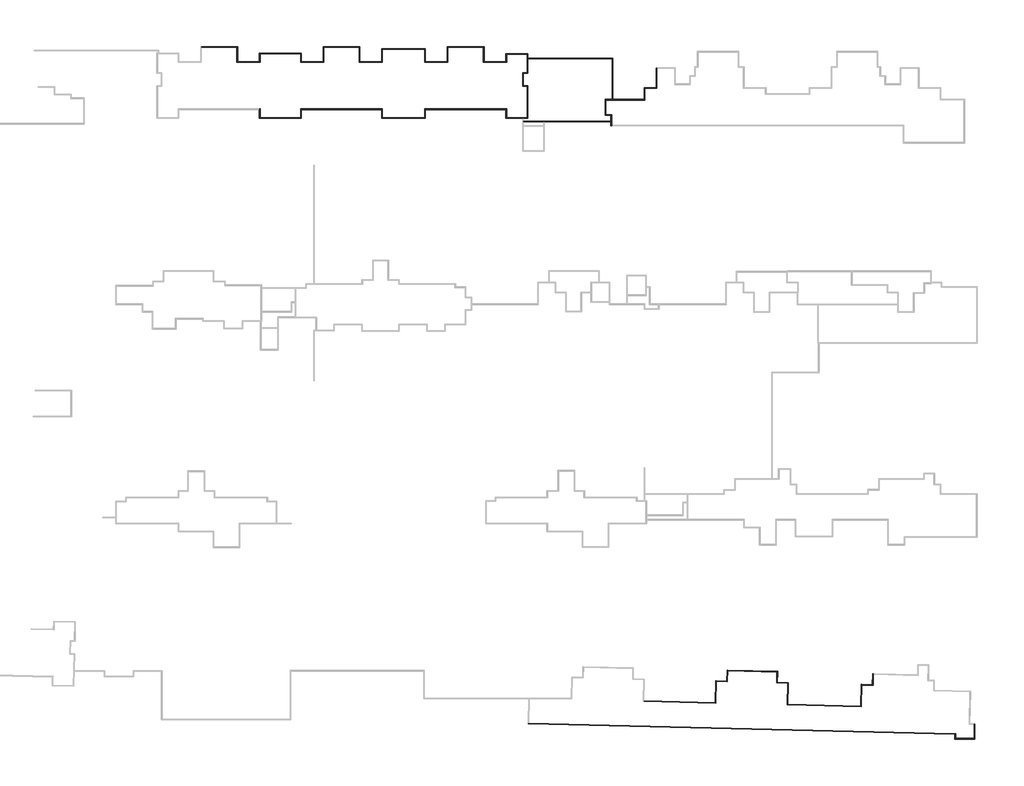
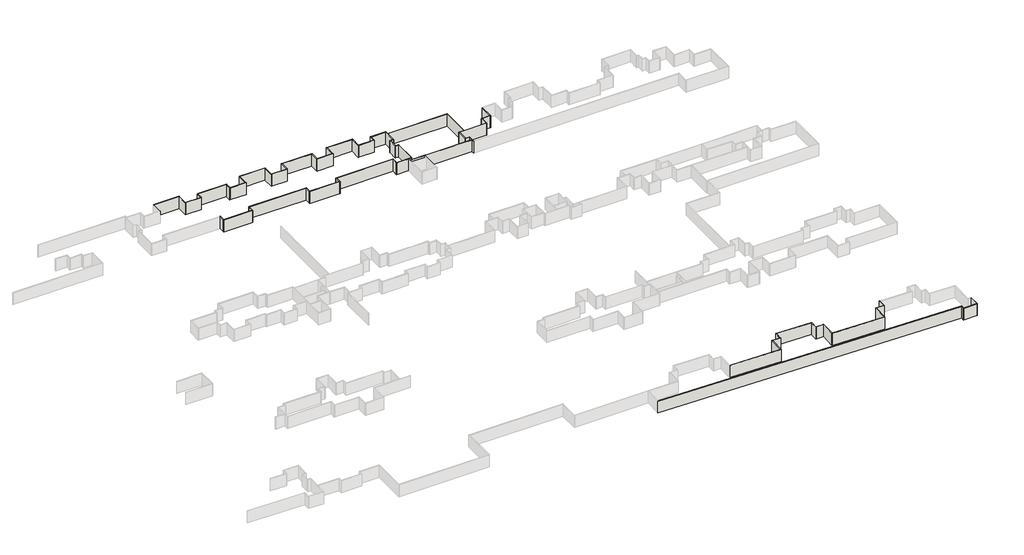
# One storey, part 6 of 8: 62 walls.
"""IFC4 building model written with IfcOpenShell, lengths in millimetres."""

import ifcopenshell
import ifcopenshell.guid

model = None  # the IFC model being written
_history = None  # IfcOwnerHistory: only IFC2X3 demands one
_inside = {}  # id of a spatial element -> (the spatial element, [elements in it])
_under = {}  # id of a project, library or spatial element -> (it, [spatial elements below it])
_declared = {}  # id of a project -> (the project, [libraries it declares])
_typed = {}  # id of a type object -> (the type object, [elements of that type])
_made_of = {}  # id of a material, layer set ... -> (it, [elements and type objects made of it])


def new_model(schema):
    """Start an empty IFC model of exactly this schema.

    Asked for "IFC4X3", IfcOpenShell would pick the latest addendum, in which some entities
    have other attributes; the version numbers below select the first issue.
    IFC2X3 requires an IfcOwnerHistory on every rooted entity: one is made here for all.
    """
    global model, _history
    if schema == "IFC4X3":
        model = ifcopenshell.file(schema_version=(4, 3, 0, 0))
    else:
        model = ifcopenshell.file(schema=schema)
    _inside.clear()
    _under.clear()
    _declared.clear()
    _typed.clear()
    _made_of.clear()
    _history = None
    if model.schema == "IFC2X3":
        org = make("IfcOrganization", Name="unknown")
        user = make(
            "IfcPersonAndOrganization",
            ThePerson=make("IfcPerson", FamilyName="unknown"),
            TheOrganization=org,
        )
        app = make(
            "IfcApplication",
            ApplicationDeveloper=org,
            Version="unknown",
            ApplicationFullName="unknown",
            ApplicationIdentifier="unknown",
        )
        _history = make(
            "IfcOwnerHistory",
            OwningUser=user,
            OwningApplication=app,
            ChangeAction="ADDED",
            CreationDate=0,
        )
    return model


def make(cls, **values):
    """One entity of the class cls with the attributes given. An attribute that is None is left unset."""
    return model.create_entity(
        cls, **{name: value for name, value in values.items() if value is not None}
    )


def rooted(cls, **values):
    """An entity with a GlobalId (a new one), such as an element, a storey or a relation."""
    return make(cls, GlobalId=ifcopenshell.guid.new(), OwnerHistory=_history, **values)


def si_unit(unit_type, name, prefix=None):
    """IfcSIUnit, for example si_unit("LENGTHUNIT", "METRE", prefix="MILLI")."""
    return make("IfcSIUnit", UnitType=unit_type, Prefix=prefix, Name=name)


def assignment(units):
    """IfcUnitAssignment: the units of a project."""
    return None if units is None else make("IfcUnitAssignment", Units=units)


def point(xyz):
    """IfcCartesianPoint."""
    return None if xyz is None else make("IfcCartesianPoint", Coordinates=xyz)


def direction(xyz):
    """IfcDirection."""
    return None if xyz is None else make("IfcDirection", DirectionRatios=xyz)


def frame(location, z_axis=None, x_axis=None):
    """IfcAxis2Placement3D, a coordinate frame: its origin and axes. An axis left out is left unset."""
    return make(
        "IfcAxis2Placement3D",
        Location=point(location),
        Axis=direction(z_axis),
        RefDirection=direction(x_axis),
    )


def origin():
    """The frame at (0, 0, 0) with its axes left unset."""
    return frame((0.0, 0.0, 0.0))


def origin_with_axes():
    """The frame at (0, 0, 0) with the z axis (0, 0, 1) and the x axis (1, 0, 0) written out."""
    return frame((0.0, 0.0, 0.0), z_axis=(0.0, 0.0, 1.0), x_axis=(1.0, 0.0, 0.0))


def place(relative_to, where):
    """IfcLocalPlacement: puts the frame where relative to a parent placement (None: the world)."""
    return make(
        "IfcLocalPlacement", PlacementRelTo=relative_to, RelativePlacement=where
    )


def context(
    kind, dimensions, precision=None, world=None, true_north=None, identifier=None
):
    """IfcGeometricRepresentationContext, for example the 3D "Model" context."""
    return make(
        "IfcGeometricRepresentationContext",
        ContextIdentifier=identifier,
        ContextType=kind,
        CoordinateSpaceDimension=dimensions,
        Precision=precision,
        WorldCoordinateSystem=world,
        TrueNorth=true_north,
    )


def project(units=None, contexts=None):
    """IfcProject with its units and contexts."""
    return rooted(
        "IfcProject",
        Name="project",
        RepresentationContexts=contexts,
        UnitsInContext=assignment(units),
    )


def spatial(cls, under=None, at=None, **own):
    """A site, building, storey or space (cls), placed at a placement, below another one or the project."""
    s = rooted(cls, ObjectPlacement=at, **own)
    if under is not None:
        _under.setdefault(under.id(), (under, []))[1].append(s)
    return s


def polyline(points):
    """IfcPolyline through the points."""
    return make("IfcPolyline", Points=[point(p) for p in points])


def outline(outer, holes=None, kind="AREA"):
    """IfcArbitraryClosedProfileDef: a profile drawn as a closed curve; with holes, ...WithVoids."""
    if holes is None:
        return make("IfcArbitraryClosedProfileDef", ProfileType=kind, OuterCurve=outer)
    return make(
        "IfcArbitraryProfileDefWithVoids",
        ProfileType=kind,
        OuterCurve=outer,
        InnerCurves=holes,
    )


def extrude(swept, where, along, depth):
    """IfcExtrudedAreaSolid: the profile swept, set in the frame where, extruded along a direction by depth."""
    return make(
        "IfcExtrudedAreaSolid",
        SweptArea=swept,
        Position=where,
        ExtrudedDirection=direction(along),
        Depth=depth,
    )


def faces_of(points, faces, orient=None, outer=None):
    """IfcFace entities. A face is a list of loops; a loop is a list of indices into points, from 0.

    orient and outer hold one flag for each loop. By default every Orientation is true, the
    first loop of a face is its IfcFaceOuterBound and the others are IfcFaceBound.
    """
    made = []
    for i, loops in enumerate(faces):
        bounds = []
        for j, loop in enumerate(loops):
            is_outer = j == 0 if outer is None else outer[i][j]
            bounds.append(
                make(
                    "IfcFaceOuterBound" if is_outer else "IfcFaceBound",
                    Bound=make("IfcPolyLoop", Polygon=[points[k] for k in loop]),
                    Orientation=True if orient is None else orient[i][j],
                )
            )
        made.append(make("IfcFace", Bounds=bounds))
    return made


def faceted_brep(points, faces, orient=None, outer=None, voids=None):
    """IfcFacetedBrep: a solid bounded by flat faces; with voids (closed shells), ...WithVoids."""
    shared = [point(p) for p in points]
    hull = make("IfcClosedShell", CfsFaces=faces_of(shared, faces, orient, outer))
    if voids is None:
        return make("IfcFacetedBrep", Outer=hull)
    return make(
        "IfcFacetedBrepWithVoids",
        Outer=hull,
        Voids=[
            make(cls, CfsFaces=faces_of(shared, fs, o, b)) for cls, fs, o, b in voids
        ],
    )


def shape(context_of_items, identifier, shape_type, items):
    """IfcShapeRepresentation: the items that make up one representation, for example the "Body"."""
    return make(
        "IfcShapeRepresentation",
        ContextOfItems=context_of_items,
        RepresentationIdentifier=identifier,
        RepresentationType=shape_type,
        Items=items,
    )


def made_of(thing, what):
    """Note that an element or type object is made of a material, layer set ...; save() writes the relation."""
    if what is not None:
        _made_of.setdefault(what.id(), (what, []))[1].append(thing)
    return thing


def element(
    cls,
    number,
    at=None,
    inside=None,
    cuts=None,
    type_object=None,
    material=None,
    context=None,
    identifier="Body",
    shape_type=None,
    held_by="IfcProductDefinitionShape",
    body=None,
    shapes=None,
    **own,
):
    """One element of the class cls, such as IfcWall. Its Tag is "e" and its number.

    at: its placement. inside: the storey or other place that contains it. cuts: it is an
    opening in that element (IfcRelVoidsElement). A single representation is given by context,
    identifier, shape_type and body (its items); several are given by shapes. held_by: the class
    of the entity that holds the representations. save() writes the other relations.
    """
    e = rooted(cls, Tag="e%d" % number, ObjectPlacement=at, **own)
    if body is not None:
        shapes = [shape(context, identifier, shape_type, body)]
    if shapes is not None:
        e.Representation = make(held_by, Representations=shapes)
    if inside is not None:
        _inside.setdefault(inside.id(), (inside, []))[1].append(e)
    if cuts is not None:
        rooted(
            "IfcRelVoidsElement", RelatingBuildingElement=cuts, RelatedOpeningElement=e
        )
    if type_object is not None:
        _typed.setdefault(type_object.id(), (type_object, []))[1].append(e)
    return made_of(e, material)


def aggregate(whole, parts):
    """IfcRelAggregates: a whole, such as a stair, and the parts it consists of."""
    return rooted("IfcRelAggregates", RelatingObject=whole, RelatedObjects=parts)


def save(model, path):
    """Write the relations noted so far, then the file.

    IfcRelAggregates (storeys below a building ...), IfcRelContainedInSpatialStructure (elements
    in a storey), IfcRelDefinesByType, IfcRelAssociatesMaterial and IfcRelDeclares: one each for
    every whole, place, type object, material and project.
    """
    for whole, parts in _under.values():
        aggregate(whole, parts)
    for where, things in _inside.values():
        rooted(
            "IfcRelContainedInSpatialStructure",
            RelatedElements=things,
            RelatingStructure=where,
        )
    for kind, things in _typed.values():
        rooted("IfcRelDefinesByType", RelatedObjects=things, RelatingType=kind)
    for what, things in _made_of.values():
        rooted("IfcRelAssociatesMaterial", RelatedObjects=things, RelatingMaterial=what)
    for by, libraries in _declared.values():
        rooted("IfcRelDeclares", RelatingContext=by, RelatedDefinitions=libraries)
    model.write(path)


model = new_model("IFC4")

# Units and contexts
model_context = context("Model", 3, world=origin())
ifc_project = project(units=[si_unit("LENGTHUNIT", "METRE", prefix="MILLI")], contexts=[model_context])

# Site, building, storey
site = spatial("IfcSite", under=ifc_project)
building = spatial("IfcBuilding", under=site)
storey = spatial("IfcBuildingStorey", under=building, Name="户型图", Elevation=0.0)

# Walls
placement = place(None, origin())
element("IfcWall", 1, ObjectType="所有墙体", at=placement, inside=storey, context=model_context, shape_type="Brep", body=[
    faceted_brep([(171910.6969649, 142127.5312689, 0.0), (178490.6969649, 142127.5312689, 0.0), (178610.6969649, 142127.5312689, 0.0), (178610.6969649, 142127.5312689, 3300.0), (178490.6969649, 142127.5312689, 3300.0), (171910.6969649, 142127.5312689, 3300.0), (171910.6969649, 142247.5312689, 0.0), (171910.6969649, 142247.5312689, 3300.0), (178610.6969649, 142247.5312689, 3300.0), (178610.6969649, 142247.5312689, 0.0)], [[[0, 1, 2, 3, 4, 5]], [[6, 7, 8, 9]], [[2, 1, 0, 6, 9]], [[5, 4, 3, 8, 7]], [[0, 5, 7, 6]], [[3, 2, 9, 8]]]),
])
element("IfcWall", 2, ObjectType="所有墙体", at=placement, inside=storey, context=model_context, shape_type="Brep", body=[
    faceted_brep([(178490.6969649, 142127.5312689, 0.0), (178490.6969649, 139327.5312675, 0.0), (178490.6969649, 139327.5312675, 3300.0), (178490.6969649, 142127.5312689, 3300.0), (178610.6969649, 142127.5312689, 0.0), (178610.6969649, 142127.5312689, 3300.0), (178610.6969649, 139447.5312675, 3300.0), (178610.6969649, 139327.5312675, 3300.0), (178610.6969649, 139327.5312675, 0.0), (178610.6969649, 139447.5312675, 0.0)], [[[0, 1, 2, 3]], [[4, 5, 6, 7, 8, 9]], [[1, 0, 4, 9, 8]], [[3, 2, 7, 6, 5]], [[0, 3, 5, 4]], [[2, 1, 8, 7]]]),
])
element("IfcWall", 3, ObjectType="所有墙体", at=placement, inside=storey, context=model_context, shape_type="Brep", body=[
    faceted_brep([(178610.6969649, 139327.5312675, 0.0), (182760.6969646, 139327.5312675, 0.0), (182760.6969646, 139327.5312675, 3300.0), (178610.6969649, 139327.5312675, 3300.0), (178610.6969649, 139447.5312675, 0.0), (178610.6969649, 139447.5312675, 3300.0), (182640.6969646, 139447.5312675, 3300.0), (182760.6969646, 139447.5312675, 3300.0), (182760.6969646, 139447.5312675, 0.0), (182640.6969646, 139447.5312675, 0.0)], [[[0, 1, 2, 3]], [[4, 5, 6, 7, 8, 9]], [[1, 0, 4, 9, 8]], [[3, 2, 7, 6, 5]], [[0, 3, 5, 4]], [[2, 1, 8, 7]]]),
])
element("IfcWall", 4, ObjectType="所有墙体", at=placement, inside=storey, context=model_context, shape_type="Brep", body=[
    faceted_brep([(182760.6969646, 139447.5312675, 0.0), (182760.6969646, 140905.0802708, 0.0), (182760.6969646, 141025.0802708, 0.0), (182760.6969646, 141025.0802708, 3300.0), (182760.6969646, 140905.0802708, 3300.0), (182760.6969646, 139447.5312675, 3300.0), (182640.6969646, 139447.5312675, 0.0), (182640.6969646, 139447.5312675, 3300.0), (182640.6969646, 141025.0802708, 3300.0), (182640.6969646, 141025.0802708, 0.0)], [[[0, 1, 2, 3, 4, 5]], [[6, 7, 8, 9]], [[2, 1, 0, 6, 9]], [[5, 4, 3, 8, 7]], [[0, 5, 7, 6]], [[3, 2, 9, 8]]]),
])
element("IfcWall", 5, ObjectType="所有墙体", at=placement, inside=storey, context=model_context, shape_type="Brep", body=[
    faceted_brep([(182760.6969646, 140905.0802708, 0.0), (190240.6969649, 140905.0802708, 0.0), (190360.6969649, 140905.0802708, 0.0), (190360.6969649, 140905.0802708, 3300.0), (190240.6969649, 140905.0802708, 3300.0), (182760.6969646, 140905.0802708, 3300.0), (182760.6969646, 141025.0802708, 0.0), (182760.6969646, 141025.0802708, 3300.0), (190360.6969649, 141025.0802708, 3300.0), (190360.6969649, 141025.0802708, 0.0)], [[[0, 1, 2, 3, 4, 5]], [[6, 7, 8, 9]], [[2, 1, 0, 6, 9]], [[5, 4, 3, 8, 7]], [[0, 5, 7, 6]], [[3, 2, 9, 8]]]),
])
element("IfcWall", 6, ObjectType="所有墙体", at=placement, inside=storey, context=model_context, shape_type="Brep", body=[
    faceted_brep([(190240.6969649, 140905.0802708, 0.0), (190240.6969649, 139327.5312675, 0.0), (190240.6969649, 139327.5312675, 3300.0), (190240.6969649, 140905.0802708, 3300.0), (190360.6969649, 140905.0802708, 0.0), (190360.6969649, 140905.0802708, 3300.0), (190360.6969649, 139447.5312675, 3300.0), (190360.6969649, 139327.5312675, 3300.0), (190360.6969649, 139327.5312675, 0.0), (190360.6969649, 139447.5312675, 0.0)], [[[0, 1, 2, 3]], [[4, 5, 6, 7, 8, 9]], [[1, 0, 4, 9, 8]], [[3, 2, 7, 6, 5]], [[0, 3, 5, 4]], [[2, 1, 8, 7]]]),
])
element("IfcWall", 7, ObjectType="所有墙体", at=placement, inside=storey, context=model_context, shape_type="Brep", body=[
    faceted_brep([(190360.6969649, 139327.5312675, 0.0), (194510.6969649, 139327.5312675, 0.0), (194510.6969649, 139327.5312675, 3300.0), (190360.6969649, 139327.5312675, 3300.0), (190360.6969649, 139447.5312675, 0.0), (190360.6969649, 139447.5312675, 3300.0), (194390.6969649, 139447.5312675, 3300.0), (194510.6969649, 139447.5312675, 3300.0), (194510.6969649, 139447.5312675, 0.0), (194390.6969649, 139447.5312675, 0.0)], [[[0, 1, 2, 3]], [[4, 5, 6, 7, 8, 9]], [[1, 0, 4, 9, 8]], [[3, 2, 7, 6, 5]], [[0, 3, 5, 4]], [[2, 1, 8, 7]]]),
])
element("IfcWall", 8, ObjectType="所有墙体", at=placement, inside=storey, context=model_context, shape_type="Brep", body=[
    faceted_brep([(194510.6969649, 139447.5312675, 0.0), (194510.6969649, 142127.5312689, 0.0), (194510.6969649, 142247.5312689, 0.0), (194510.6969649, 142247.5312689, 3300.0), (194510.6969649, 142127.5312689, 3300.0), (194510.6969649, 139447.5312675, 3300.0), (194390.6969649, 139447.5312675, 0.0), (194390.6969649, 139447.5312675, 3300.0), (194390.6969649, 142247.5312689, 3300.0), (194390.6969649, 142247.5312689, 0.0)], [[[0, 1, 2, 3, 4, 5]], [[6, 7, 8, 9]], [[2, 1, 0, 6, 9]], [[5, 4, 3, 8, 7]], [[0, 5, 7, 6]], [[3, 2, 9, 8]]]),
])
element("IfcWall", 9, ObjectType="所有墙体", at=placement, inside=storey, context=model_context, shape_type="Brep", body=[
    faceted_brep([(194510.6969649, 142127.5312689, 0.0), (201090.6969649, 142127.5312689, 0.0), (201210.6969649, 142127.5312689, 0.0), (201210.6969649, 142127.5312689, 3300.0), (201090.6969649, 142127.5312689, 3300.0), (194510.6969649, 142127.5312689, 3300.0), (194510.6969649, 142247.5312689, 0.0), (194510.6969649, 142247.5312689, 3300.0), (201210.6969649, 142247.5312689, 3300.0), (201210.6969649, 142247.5312689, 0.0)], [[[0, 1, 2, 3, 4, 5]], [[6, 7, 8, 9]], [[2, 1, 0, 6, 9]], [[5, 4, 3, 8, 7]], [[0, 5, 7, 6]], [[3, 2, 9, 8]]]),
])
element("IfcWall", 10, ObjectType="所有墙体", at=placement, inside=storey, context=model_context, shape_type="Brep", body=[
    faceted_brep([(201090.6969649, 142127.5312689, 0.0), (201090.6969649, 139327.5312675, 0.0), (201090.6969649, 139327.5312675, 3300.0), (201090.6969649, 142127.5312689, 3300.0), (201210.6969649, 142127.5312689, 0.0), (201210.6969649, 142127.5312689, 3300.0), (201210.6969649, 139447.5312675, 3300.0), (201210.6969649, 139327.5312675, 3300.0), (201210.6969649, 139327.5312675, 0.0), (201210.6969649, 139447.5312675, 0.0)], [[[0, 1, 2, 3]], [[4, 5, 6, 7, 8, 9]], [[1, 0, 4, 9, 8]], [[3, 2, 7, 6, 5]], [[0, 3, 5, 4]], [[2, 1, 8, 7]]]),
])
element("IfcWall", 11, ObjectType="所有墙体", at=placement, inside=storey, context=model_context, shape_type="Brep", body=[
    faceted_brep([(201210.6969649, 139327.5312675, 0.0), (205360.6969646, 139327.5312675, 0.0), (205360.6969646, 139327.5312675, 3300.0), (201210.6969649, 139327.5312675, 3300.0), (201210.6969649, 139447.5312675, 0.0), (201210.6969649, 139447.5312675, 3300.0), (205240.6969646, 139447.5312675, 3300.0), (205360.6969646, 139447.5312675, 3300.0), (205360.6969646, 139447.5312675, 0.0), (205240.6969646, 139447.5312675, 0.0)], [[[0, 1, 2, 3]], [[4, 5, 6, 7, 8, 9]], [[1, 0, 4, 9, 8]], [[3, 2, 7, 6, 5]], [[0, 3, 5, 4]], [[2, 1, 8, 7]]]),
])
element("IfcWall", 12, ObjectType="所有墙体", at=placement, inside=storey, context=model_context, shape_type="Brep", body=[
    faceted_brep([(205360.6969646, 139447.5312675, 0.0), (205360.6969646, 141727.5312675, 0.0), (205360.6969646, 141847.5312675, 0.0), (205360.6969646, 141847.5312675, 3300.0), (205360.6969646, 141727.5312675, 3300.0), (205360.6969646, 139447.5312675, 3300.0), (205240.6969646, 139447.5312675, 0.0), (205240.6969646, 139447.5312675, 3300.0), (205240.6969646, 141847.5312675, 3300.0), (205240.6969646, 141847.5312675, 0.0)], [[[0, 1, 2, 3, 4, 5]], [[6, 7, 8, 9]], [[2, 1, 0, 6, 9]], [[5, 4, 3, 8, 7]], [[0, 5, 7, 6]], [[3, 2, 9, 8]]]),
])
element("IfcWall", 13, ObjectType="所有墙体", at=placement, inside=storey, context=model_context, shape_type="Brep", body=[
    faceted_brep([(205360.6969646, 141727.5312675, 0.0), (213140.6969649, 141727.5312675, 0.0), (213260.6969649, 141727.5312675, 0.0), (213260.6969649, 141727.5312675, 3300.0), (213140.6969649, 141727.5312675, 3300.0), (205360.6969646, 141727.5312675, 3300.0), (205360.6969646, 141847.5312675, 0.0), (205360.6969646, 141847.5312675, 3300.0), (213260.6969649, 141847.5312675, 3300.0), (213260.6969649, 141847.5312675, 0.0)], [[[0, 1, 2, 3, 4, 5]], [[6, 7, 8, 9]], [[2, 1, 0, 6, 9]], [[5, 4, 3, 8, 7]], [[0, 5, 7, 6]], [[3, 2, 9, 8]]]),
])
element("IfcWall", 14, ObjectType="所有墙体", at=placement, inside=storey, context=model_context, shape_type="Brep", body=[
    faceted_brep([(213140.6969649, 141727.5312675, 0.0), (213140.6969649, 139327.5312675, 0.0), (213140.6969649, 139327.5312675, 3300.0), (213140.6969649, 141727.5312675, 3300.0), (213260.6969649, 141727.5312675, 0.0), (213260.6969649, 141727.5312675, 3300.0), (213260.6969649, 139447.5312675, 3300.0), (213260.6969649, 139327.5312675, 3300.0), (213260.6969649, 139327.5312675, 0.0), (213260.6969649, 139447.5312675, 0.0)], [[[0, 1, 2, 3]], [[4, 5, 6, 7, 8, 9]], [[1, 0, 4, 9, 8]], [[3, 2, 7, 6, 5]], [[0, 3, 5, 4]], [[2, 1, 8, 7]]]),
])
element("IfcWall", 15, ObjectType="所有墙体", at=placement, inside=storey, context=model_context, shape_type="Brep", body=[
    faceted_brep([(213260.6969649, 139327.5312675, 0.0), (217410.6969649, 139327.5312675, 0.0), (217410.6969649, 139327.5312675, 3300.0), (213260.6969649, 139327.5312675, 3300.0), (213260.6969649, 139447.5312675, 0.0), (213260.6969649, 139447.5312675, 3300.0), (217290.6969649, 139447.5312675, 3300.0), (217410.6969649, 139447.5312675, 3300.0), (217410.6969649, 139447.5312675, 0.0), (217290.6969649, 139447.5312675, 0.0)], [[[0, 1, 2, 3]], [[4, 5, 6, 7, 8, 9]], [[1, 0, 4, 9, 8]], [[3, 2, 7, 6, 5]], [[0, 3, 5, 4]], [[2, 1, 8, 7]]]),
])
element("IfcWall", 16, ObjectType="所有墙体", at=placement, inside=storey, context=model_context, shape_type="Brep", body=[
    faceted_brep([(217410.6969649, 139447.5312675, 0.0), (217410.6969649, 142127.5312689, 0.0), (217410.6969649, 142247.5312689, 0.0), (217410.6969649, 142247.5312689, 3300.0), (217410.6969649, 142127.5312689, 3300.0), (217410.6969649, 139447.5312675, 3300.0), (217290.6969649, 139447.5312675, 0.0), (217290.6969649, 139447.5312675, 3300.0), (217290.6969649, 142247.5312689, 3300.0), (217290.6969649, 142247.5312689, 0.0)], [[[0, 1, 2, 3, 4, 5]], [[6, 7, 8, 9]], [[2, 1, 0, 6, 9]], [[5, 4, 3, 8, 7]], [[0, 5, 7, 6]], [[3, 2, 9, 8]]]),
])
element("IfcWall", 17, ObjectType="所有墙体", at=placement, inside=storey, context=model_context, shape_type="Brep", body=[
    faceted_brep([(217410.6969649, 142127.5312689, 0.0), (223990.6969649, 142127.5312689, 0.0), (224110.6969649, 142127.5312689, 0.0), (224110.6969649, 142127.5312689, 3300.0), (223990.6969649, 142127.5312689, 3300.0), (217410.6969649, 142127.5312689, 3300.0), (217410.6969649, 142247.5312689, 0.0), (217410.6969649, 142247.5312689, 3300.0), (224110.6969649, 142247.5312689, 3300.0), (224110.6969649, 142247.5312689, 0.0)], [[[0, 1, 2, 3, 4, 5]], [[6, 7, 8, 9]], [[2, 1, 0, 6, 9]], [[5, 4, 3, 8, 7]], [[0, 5, 7, 6]], [[3, 2, 9, 8]]]),
])
element("IfcWall", 18, ObjectType="所有墙体", at=placement, inside=storey, context=model_context, shape_type="Brep", body=[
    faceted_brep([(223990.6969649, 142127.5312689, 0.0), (223990.6969649, 139327.5312675, 0.0), (223990.6969649, 139327.5312675, 3300.0), (223990.6969649, 142127.5312689, 3300.0), (224110.6969649, 142127.5312689, 0.0), (224110.6969649, 142127.5312689, 3300.0), (224110.6969649, 139447.5312675, 3300.0), (224110.6969649, 139327.5312675, 3300.0), (224110.6969649, 139327.5312675, 0.0), (224110.6969649, 139447.5312675, 0.0)], [[[0, 1, 2, 3]], [[4, 5, 6, 7, 8, 9]], [[1, 0, 4, 9, 8]], [[3, 2, 7, 6, 5]], [[0, 3, 5, 4]], [[2, 1, 8, 7]]]),
])
element("IfcWall", 19, ObjectType="所有墙体", at=placement, inside=storey, context=model_context, shape_type="Brep", body=[
    faceted_brep([(224110.6969649, 139327.5312675, 0.0), (228260.6969646, 139327.5312675, 0.0), (228260.6969646, 139327.5312675, 3300.0), (224110.6969649, 139327.5312675, 3300.0), (224110.6969649, 139447.5312675, 0.0), (224110.6969649, 139447.5312675, 3300.0), (228140.6969646, 139447.5312675, 3300.0), (228260.6969646, 139447.5312675, 3300.0), (228260.6969646, 139447.5312675, 0.0), (228140.6969646, 139447.5312675, 0.0)], [[[0, 1, 2, 3]], [[4, 5, 6, 7, 8, 9]], [[1, 0, 4, 9, 8]], [[3, 2, 7, 6, 5]], [[0, 3, 5, 4]], [[2, 1, 8, 7]]]),
])
element("IfcWall", 20, ObjectType="所有墙体", at=placement, inside=storey, context=model_context, shape_type="Brep", body=[
    faceted_brep([(228260.6969646, 139447.5312675, 0.0), (228260.6969646, 140827.5312675, 0.0), (228260.6969646, 140947.5312675, 0.0), (228260.6969646, 140947.5312675, 3300.0), (228260.6969646, 140827.5312675, 3300.0), (228260.6969646, 139447.5312675, 3300.0), (228140.6969646, 139447.5312675, 0.0), (228140.6969646, 139447.5312675, 3300.0), (228140.6969646, 140947.5312675, 3300.0), (228140.6969646, 140947.5312675, 0.0)], [[[0, 1, 2, 3, 4, 5]], [[6, 7, 8, 9]], [[2, 1, 0, 6, 9]], [[5, 4, 3, 8, 7]], [[0, 5, 7, 6]], [[3, 2, 9, 8]]]),
])
element("IfcWall", 21, ObjectType="所有墙体", at=placement, inside=storey, context=model_context, shape_type="Brep", body=[
    faceted_brep([(228260.6969646, 140827.5312675, 0.0), (232040.6969642, 140827.5312675, 0.0), (232160.6969642, 140827.5312675, 0.0), (232160.6969642, 140827.5312675, 3300.0), (232040.6969642, 140827.5312675, 3300.0), (228260.6969646, 140827.5312675, 3300.0), (228260.6969646, 140947.5312675, 0.0), (228260.6969646, 140947.5312675, 3300.0), (232160.6969642, 140947.5312675, 3300.0), (232160.6969642, 140947.5312675, 0.0)], [[[0, 1, 2, 3, 4, 5]], [[6, 7, 8, 9]], [[2, 1, 0, 6, 9]], [[5, 4, 3, 8, 7]], [[0, 5, 7, 6]], [[3, 2, 9, 8]]]),
])
element("IfcWall", 22, ObjectType="所有墙体", at=placement, inside=storey, context=model_context, shape_type="Brep", body=[
    faceted_brep([(232040.6969642, 140827.5312675, 0.0), (232040.6969642, 137447.5312675, 0.0), (232040.6969642, 137327.5312675, 0.0), (232040.6969642, 137327.5312675, 3300.0), (232040.6969642, 137447.5312675, 3300.0), (232040.6969642, 140827.5312675, 3300.0), (232160.6969642, 140827.5312675, 0.0), (232160.6969642, 140827.5312675, 3300.0), (232160.6969642, 140107.5312675, 3300.0), (232160.6969642, 139987.5312675, 3300.0), (232160.6969642, 137327.5312675, 3300.0), (232160.6969642, 137327.5312675, 0.0), (232160.6969642, 139987.5312675, 0.0), (232160.6969642, 140107.5312675, 0.0)], [[[0, 1, 2, 3, 4, 5]], [[6, 7, 8, 9, 10, 11, 12, 13]], [[2, 1, 0, 6, 13, 12, 11]], [[5, 4, 3, 10, 9, 8, 7]], [[0, 5, 7, 6]], [[3, 2, 11, 10]]]),
])
element("IfcWall", 23, ObjectType="所有墙体", at=placement, inside=storey, context=model_context, shape_type="Brep", body=[
    faceted_brep([(232040.6969642, 137447.5312675, 0.0), (231240.6969648, 137447.5312675, 0.0), (231240.6969648, 137447.5312675, 3300.0), (232040.6969642, 137447.5312675, 3300.0), (232040.6969642, 137327.5312675, 0.0), (232040.6969642, 137327.5312675, 3300.0), (231360.6969648, 137327.5312675, 3300.0), (231240.6969648, 137327.5312675, 3300.0), (231240.6969648, 137327.5312675, 0.0), (231360.6969648, 137327.5312675, 0.0)], [[[0, 1, 2, 3]], [[4, 5, 6, 7, 8, 9]], [[1, 0, 4, 9, 8]], [[3, 2, 7, 6, 5]], [[0, 3, 5, 4]], [[2, 1, 8, 7]]]),
])
element("IfcWall", 24, ObjectType="所有墙体", at=placement, inside=storey, context=model_context, shape_type="Brep", body=[
    faceted_brep([(231240.6969648, 137327.5312675, 0.0), (231240.6969648, 134927.5312611, 0.0), (231240.6969648, 134927.5312611, 3300.0), (231240.6969648, 137327.5312675, 3300.0), (231360.6969648, 137327.5312675, 0.0), (231360.6969648, 137327.5312675, 3300.0), (231360.6969648, 135047.5312611, 3300.0), (231360.6969648, 134927.5312611, 3300.0), (231360.6969648, 134927.5312611, 0.0), (231360.6969648, 135047.5312611, 0.0)], [[[0, 1, 2, 3]], [[4, 5, 6, 7, 8, 9]], [[1, 0, 4, 9, 8]], [[3, 2, 7, 6, 5]], [[0, 3, 5, 4]], [[2, 1, 8, 7]]]),
])
element("IfcWall", 25, ObjectType="所有墙体", at=placement, inside=storey, context=model_context, shape_type="Brep", body=[
    faceted_brep([(231360.6969648, 134927.5312611, 0.0), (232040.6969642, 134927.5312611, 0.0), (232160.6969642, 134927.5312611, 0.0), (232160.6969642, 134927.5312611, 3300.0), (232040.6969642, 134927.5312611, 3300.0), (231360.6969648, 134927.5312611, 3300.0), (231360.6969648, 135047.5312611, 0.0), (231360.6969648, 135047.5312611, 3300.0), (232160.6969642, 135047.5312611, 3300.0), (232160.6969642, 135047.5312611, 0.0)], [[[0, 1, 2, 3, 4, 5]], [[6, 7, 8, 9]], [[2, 1, 0, 6, 9]], [[5, 4, 3, 8, 7]], [[0, 5, 7, 6]], [[3, 2, 9, 8]]]),
])
element("IfcWall", 26, ObjectType="所有墙体", at=placement, inside=storey, context=model_context, shape_type="Brep", body=[
    faceted_brep([(232040.6969642, 134927.5312611, 0.0), (232040.6969642, 129147.5312684, 0.0), (232040.6969642, 129027.5312684, 0.0), (232040.6969642, 129027.5312684, 3300.0), (232040.6969642, 129147.5312684, 3300.0), (232040.6969642, 134927.5312611, 3300.0), (232160.6969642, 134927.5312611, 0.0), (232160.6969642, 134927.5312611, 3300.0), (232160.6969642, 129027.5312684, 3300.0), (232160.6969642, 129027.5312684, 0.0)], [[[0, 1, 2, 3, 4, 5]], [[6, 7, 8, 9]], [[2, 1, 0, 6, 9]], [[5, 4, 3, 8, 7]], [[0, 5, 7, 6]], [[3, 2, 9, 8]]]),
])
element("IfcWall", 27, ObjectType="所有墙体", at=placement, inside=storey, context=model_context, shape_type="Brep", body=[
    faceted_brep([(232040.6969642, 129147.5312684, 0.0), (228260.6969646, 129147.5312684, 0.0), (228140.6969646, 129147.5312684, 0.0), (228140.6969646, 129147.5312684, 3300.0), (228260.6969646, 129147.5312684, 3300.0), (232040.6969642, 129147.5312684, 3300.0), (232040.6969642, 129027.5312684, 0.0), (232040.6969642, 129027.5312684, 3300.0), (231369.8041277, 129027.5312684, 3300.0), (231249.8041277, 129027.5312684, 3300.0), (228140.6969646, 129027.5312684, 3300.0), (228140.6969646, 129027.5312684, 0.0), (231249.8041277, 129027.5312684, 0.0), (231369.8041277, 129027.5312684, 0.0)], [[[0, 1, 2, 3, 4, 5]], [[6, 7, 8, 9, 10, 11, 12, 13]], [[2, 1, 0, 6, 13, 12, 11]], [[5, 4, 3, 10, 9, 8, 7]], [[0, 5, 7, 6]], [[3, 2, 11, 10]]]),
])
element("IfcWall", 28, ObjectType="所有墙体", at=placement, inside=storey, context=model_context, shape_type="Brep", body=[
    faceted_brep([(228260.6969646, 129147.5312684, 0.0), (228260.6969646, 130747.5312684, 0.0), (228260.6969646, 130747.5312684, 3300.0), (228260.6969646, 129147.5312684, 3300.0), (228140.6969646, 129147.5312684, 0.0), (228140.6969646, 129147.5312684, 3300.0), (228140.6969646, 130627.5312684, 3300.0), (228140.6969646, 130747.5312684, 3300.0), (228140.6969646, 130747.5312684, 0.0), (228140.6969646, 130627.5312684, 0.0)], [[[0, 1, 2, 3]], [[4, 5, 6, 7, 8, 9]], [[1, 0, 4, 9, 8]], [[3, 2, 7, 6, 5]], [[0, 3, 5, 4]], [[2, 1, 8, 7]]]),
])
element("IfcWall", 29, ObjectType="所有墙体", at=placement, inside=storey, context=model_context, shape_type="Brep", body=[
    faceted_brep([(228140.6969646, 130747.5312684, 0.0), (213140.6969649, 130747.5312684, 0.0), (213140.6969649, 130747.5312684, 3300.0), (228140.6969646, 130747.5312684, 3300.0), (228140.6969646, 130627.5312684, 0.0), (228140.6969646, 130627.5312684, 3300.0), (213260.6969649, 130627.5312684, 3300.0), (213140.6969649, 130627.5312684, 3300.0), (213140.6969649, 130627.5312684, 0.0), (213260.6969649, 130627.5312684, 0.0)], [[[0, 1, 2, 3]], [[4, 5, 6, 7, 8, 9]], [[1, 0, 4, 9, 8]], [[3, 2, 7, 6, 5]], [[0, 3, 5, 4]], [[2, 1, 8, 7]]]),
])
element("IfcWall", 30, ObjectType="所有墙体", at=placement, inside=storey, context=model_context, shape_type="Brep", body=[
    faceted_brep([(213140.6969649, 130627.5312684, 0.0), (213140.6969649, 129147.5312684, 0.0), (213140.6969649, 129027.5312684, 0.0), (213140.6969649, 129027.5312684, 3300.0), (213140.6969649, 129147.5312684, 3300.0), (213140.6969649, 130627.5312684, 3300.0), (213260.6969649, 130627.5312684, 0.0), (213260.6969649, 130627.5312684, 3300.0), (213260.6969649, 129027.5312684, 3300.0), (213260.6969649, 129027.5312684, 0.0)], [[[0, 1, 2, 3, 4, 5]], [[6, 7, 8, 9]], [[2, 1, 0, 6, 9]], [[5, 4, 3, 8, 7]], [[0, 5, 7, 6]], [[3, 2, 9, 8]]]),
])
element("IfcWall", 31, ObjectType="所有墙体", at=placement, inside=storey, context=model_context, shape_type="Brep", body=[
    faceted_brep([(213140.6969649, 129147.5312684, 0.0), (205360.6969646, 129147.5312684, 0.0), (205240.6969646, 129147.5312684, 0.0), (205240.6969646, 129147.5312684, 3300.0), (205360.6969646, 129147.5312684, 3300.0), (213140.6969649, 129147.5312684, 3300.0), (213140.6969649, 129027.5312684, 0.0), (213140.6969649, 129027.5312684, 3300.0), (205240.6969646, 129027.5312684, 3300.0), (205240.6969646, 129027.5312684, 0.0)], [[[0, 1, 2, 3, 4, 5]], [[6, 7, 8, 9]], [[2, 1, 0, 6, 9]], [[5, 4, 3, 8, 7]], [[0, 5, 7, 6]], [[3, 2, 9, 8]]]),
])
element("IfcWall", 32, ObjectType="所有墙体", at=placement, inside=storey, context=model_context, shape_type="Brep", body=[
    faceted_brep([(205360.6969646, 129147.5312684, 0.0), (205360.6969646, 130747.5312684, 0.0), (205360.6969646, 130747.5312684, 3300.0), (205360.6969646, 129147.5312684, 3300.0), (205240.6969646, 129147.5312684, 0.0), (205240.6969646, 129147.5312684, 3300.0), (205240.6969646, 130627.5312684, 3300.0), (205240.6969646, 130747.5312684, 3300.0), (205240.6969646, 130747.5312684, 0.0), (205240.6969646, 130627.5312684, 0.0)], [[[0, 1, 2, 3]], [[4, 5, 6, 7, 8, 9]], [[1, 0, 4, 9, 8]], [[3, 2, 7, 6, 5]], [[0, 3, 5, 4]], [[2, 1, 8, 7]]]),
])
element("IfcWall", 33, ObjectType="所有墙体", at=placement, inside=storey, context=model_context, shape_type="Brep", body=[
    faceted_brep([(205240.6969646, 130747.5312684, 0.0), (190240.6969649, 130747.5312684, 0.0), (190240.6969649, 130747.5312684, 3300.0), (205240.6969646, 130747.5312684, 3300.0), (205240.6969646, 130627.5312684, 0.0), (205240.6969646, 130627.5312684, 3300.0), (190360.6969649, 130627.5312684, 3300.0), (190240.6969649, 130627.5312684, 3300.0), (190240.6969649, 130627.5312684, 0.0), (190360.6969649, 130627.5312684, 0.0)], [[[0, 1, 2, 3]], [[4, 5, 6, 7, 8, 9]], [[1, 0, 4, 9, 8]], [[3, 2, 7, 6, 5]], [[0, 3, 5, 4]], [[2, 1, 8, 7]]]),
])
element("IfcWall", 34, ObjectType="所有墙体", at=placement, inside=storey, context=model_context, shape_type="Brep", body=[
    faceted_brep([(190240.6969649, 130627.5312684, 0.0), (190240.6969649, 129147.5312684, 0.0), (190240.6969649, 129027.5312684, 0.0), (190240.6969649, 129027.5312684, 3300.0), (190240.6969649, 129147.5312684, 3300.0), (190240.6969649, 130627.5312684, 3300.0), (190360.6969649, 130627.5312684, 0.0), (190360.6969649, 130627.5312684, 3300.0), (190360.6969649, 129027.5312684, 3300.0), (190360.6969649, 129027.5312684, 0.0)], [[[0, 1, 2, 3, 4, 5]], [[6, 7, 8, 9]], [[2, 1, 0, 6, 9]], [[5, 4, 3, 8, 7]], [[0, 5, 7, 6]], [[3, 2, 9, 8]]]),
])
element("IfcWall", 35, ObjectType="所有墙体", at=placement, inside=storey, context=model_context, shape_type="Brep", body=[
    faceted_brep([(190240.6969649, 129147.5312684, 0.0), (182760.6969646, 129147.5312684, 0.0), (182640.6969646, 129147.5312684, 0.0), (182640.6969646, 129147.5312684, 3300.0), (182760.6969646, 129147.5312684, 3300.0), (190240.6969649, 129147.5312684, 3300.0), (190240.6969649, 129027.5312684, 0.0), (190240.6969649, 129027.5312684, 3300.0), (182640.6969646, 129027.5312684, 3300.0), (182640.6969646, 129027.5312684, 0.0)], [[[0, 1, 2, 3, 4, 5]], [[6, 7, 8, 9]], [[2, 1, 0, 6, 9]], [[5, 4, 3, 8, 7]], [[0, 5, 7, 6]], [[3, 2, 9, 8]]]),
])
element("IfcWall", 36, ObjectType="所有墙体", at=placement, inside=storey, context=model_context, shape_type="Brep", body=[
    faceted_brep([(182760.6969646, 129147.5312684, 0.0), (182760.6969646, 130747.5312684, 0.0), (182760.6969646, 130747.5312684, 3300.0), (182760.6969646, 129147.5312684, 3300.0), (182640.6969646, 129147.5312684, 0.0), (182640.6969646, 129147.5312684, 3300.0), (182640.6969646, 130627.5312684, 3300.0), (182640.6969646, 130747.5312684, 3300.0), (182640.6969646, 130747.5312684, 0.0), (182640.6969646, 130627.5312684, 0.0)], [[[0, 1, 2, 3]], [[4, 5, 6, 7, 8, 9]], [[1, 0, 4, 9, 8]], [[3, 2, 7, 6, 5]], [[0, 3, 5, 4]], [[2, 1, 8, 7]]]),
])
element("IfcWall", 37, ObjectType="所有墙体", at=placement, inside=storey, context=model_context, shape_type="Brep", body=[
    faceted_brep([(253581.2528793, 21363.7654177, 0.0), (266877.2414257, 21037.1332476, 0.0), (266877.2414257, 21037.1332476, 3300.0), (253581.2528793, 21363.7654177, 3300.0), (253584.1999365, 21483.7292241, 0.0), (253584.1999365, 21483.7292241, 3300.0), (266760.2246764, 21160.0441112, 3300.0), (266880.1884829, 21157.097054, 3300.0), (266880.1884829, 21157.097054, 0.0), (266760.2246764, 21160.0441112, 0.0)], [[[0, 1, 2, 3]], [[4, 5, 6, 7, 8, 9]], [[1, 0, 4, 9, 8]], [[3, 2, 7, 6, 5]], [[0, 3, 5, 4]], [[2, 1, 8, 7]]]),
])
element("IfcWall", 38, ObjectType="所有墙体", at=placement, inside=storey, context=model_context, shape_type="Brep", body=[
    faceted_brep([(266880.1884829, 21157.097054, 0.0), (266975.9558887, 25055.4342273, 0.0), (266978.9029458, 25175.3980337, 0.0), (266978.9029458, 25175.3980337, 3300.0), (266975.9558887, 25055.4342273, 3300.0), (266880.1884829, 21157.097054, 3300.0), (266760.2246764, 21160.0441112, 0.0), (266760.2246764, 21160.0441112, 3300.0), (266858.9391394, 25178.3450909, 3300.0), (266858.9391394, 25178.3450909, 0.0)], [[[0, 1, 2, 3, 4, 5]], [[6, 7, 8, 9]], [[2, 1, 0, 6, 9]], [[5, 4, 3, 8, 7]], [[0, 5, 7, 6]], [[3, 2, 9, 8]]]),
])
element("IfcWall", 39, ObjectType="所有墙体", at=placement, inside=storey, context=model_context, shape_type="Brep", body=[
    faceted_brep([(266975.9558887, 25055.4342273, 0.0), (269035.3345658, 25004.8430791, 0.0), (269035.3345658, 25004.8430791, 3300.0), (266975.9558887, 25055.4342273, 3300.0), (266978.9029458, 25175.3980337, 0.0), (266978.9029458, 25175.3980337, 3300.0), (268918.3178165, 25127.7539427, 3300.0), (269038.2816229, 25124.8068856, 3300.0), (269038.2816229, 25124.8068856, 0.0), (268918.3178165, 25127.7539427, 0.0)], [[[0, 1, 2, 3]], [[4, 5, 6, 7, 8, 9]], [[1, 0, 4, 9, 8]], [[3, 2, 7, 6, 5]], [[0, 3, 5, 4]], [[2, 1, 8, 7]]]),
])
element("IfcWall", 40, ObjectType="所有墙体", at=placement, inside=storey, context=model_context, shape_type="Brep", body=[
    faceted_brep([(269038.2816229, 25124.8068856, 0.0), (269084.4408606, 27003.778863, 0.0), (269087.3879177, 27123.7426694, 0.0), (269087.3879177, 27123.7426694, 3300.0), (269084.4408606, 27003.778863, 3300.0), (269038.2816229, 25124.8068856, 3300.0), (268918.3178165, 25127.7539427, 0.0), (268918.3178165, 25127.7539427, 3300.0), (268967.4241113, 27126.6897266, 3300.0), (268967.4241113, 27126.6897266, 0.0)], [[[0, 1, 2, 3, 4, 5]], [[6, 7, 8, 9]], [[2, 1, 0, 6, 9]], [[5, 4, 3, 8, 7]], [[0, 5, 7, 6]], [[3, 2, 9, 8]]]),
])
element("IfcWall", 41, ObjectType="所有墙体", at=placement, inside=storey, context=model_context, shape_type="Brep", body=[
    faceted_brep([(269084.4408606, 27003.778863, 0.0), (278161.702214, 26780.7848702, 0.0), (278281.6660205, 26777.837813, 0.0), (278281.6660205, 26777.837813, 3300.0), (278161.702214, 26780.7848702, 3300.0), (269084.4408606, 27003.778863, 3300.0), (269087.3879177, 27123.7426694, 0.0), (269087.3879177, 27123.7426694, 3300.0), (278284.6130776, 26897.8016195, 3300.0), (278284.6130776, 26897.8016195, 0.0)], [[[0, 1, 2, 3, 4, 5]], [[6, 7, 8, 9]], [[2, 1, 0, 6, 9]], [[5, 4, 3, 8, 7]], [[0, 5, 7, 6]], [[3, 2, 9, 8]]]),
])
element("IfcWall", 42, ObjectType="所有墙体", at=placement, inside=storey, context=model_context, shape_type="Brep", body=[
    faceted_brep([(278161.702214, 26780.7848702, 0.0), (278112.5962349, 24781.8619362, 0.0), (278112.5962349, 24781.8619362, 3300.0), (278161.702214, 26780.7848702, 3300.0), (278281.6660205, 26777.837813, 0.0), (278281.6660205, 26777.837813, 3300.0), (278235.5070985, 24898.8786854, 3300.0), (278232.5600414, 24778.914879, 3300.0), (278232.5600414, 24778.914879, 0.0), (278235.5070985, 24898.8786854, 0.0)], [[[0, 1, 2, 3]], [[4, 5, 6, 7, 8, 9]], [[1, 0, 4, 9, 8]], [[3, 2, 7, 6, 5]], [[0, 3, 5, 4]], [[2, 1, 8, 7]]]),
])
element("IfcWall", 43, ObjectType="所有墙体", at=placement, inside=storey, context=model_context, shape_type="Brep", body=[
    faceted_brep([(278232.5600414, 24778.914879, 0.0), (280151.1308314, 24731.7828483, 0.0), (280271.0946379, 24728.8357911, 0.0), (280271.0946379, 24728.8357911, 3300.0), (280151.1308314, 24731.7828483, 3300.0), (278232.5600414, 24778.914879, 3300.0), (278235.5070985, 24898.8786854, 0.0), (278235.5070985, 24898.8786854, 3300.0), (280274.041695, 24848.7995976, 3300.0), (280274.041695, 24848.7995976, 0.0)], [[[0, 1, 2, 3, 4, 5]], [[6, 7, 8, 9]], [[2, 1, 0, 6, 9]], [[5, 4, 3, 8, 7]], [[0, 5, 7, 6]], [[3, 2, 9, 8]]]),
])
element("IfcWall", 44, ObjectType="所有墙体", at=placement, inside=storey, context=model_context, shape_type="Brep", body=[
    faceted_brep([(280151.1308314, 24731.7828483, 0.0), (280052.8955923, 20732.9893005, 0.0), (280052.8955923, 20732.9893005, 3300.0), (280151.1308314, 24731.7828483, 3300.0), (280271.0946379, 24728.8357911, 0.0), (280271.0946379, 24728.8357911, 3300.0), (280175.8064559, 20850.0060498, 3300.0), (280172.8593987, 20730.0422433, 3300.0), (280172.8593987, 20730.0422433, 0.0), (280175.8064559, 20850.0060498, 0.0)], [[[0, 1, 2, 3]], [[4, 5, 6, 7, 8, 9]], [[1, 0, 4, 9, 8]], [[3, 2, 7, 6, 5]], [[0, 3, 5, 4]], [[2, 1, 8, 7]]]),
])
element("IfcWall", 45, ObjectType="所有墙体", at=placement, inside=storey, context=model_context, shape_type="Brep", body=[
    faceted_brep([(280172.8593987, 20730.0422433, 0.0), (293768.7574612, 20396.0424304, 0.0), (293768.7574612, 20396.0424304, 3300.0), (280172.8593987, 20730.0422433, 3300.0), (280175.8064559, 20850.0060498, 0.0), (280175.8064559, 20850.0060498, 3300.0), (293651.740712, 20518.953294, 3300.0), (293771.7045184, 20516.0062368, 3300.0), (293771.7045184, 20516.0062368, 0.0), (293651.740712, 20518.953294, 0.0)], [[[0, 1, 2, 3]], [[4, 5, 6, 7, 8, 9]], [[1, 0, 4, 9, 8]], [[3, 2, 7, 6, 5]], [[0, 3, 5, 4]], [[2, 1, 8, 7]]]),
])
element("IfcWall", 46, ObjectType="所有墙体", at=placement, inside=storey, context=model_context, shape_type="Brep", body=[
    faceted_brep([(293771.7045184, 20516.0062368, 0.0), (293866.9910313, 24394.7680372, 0.0), (293869.9380884, 24514.7318436, 0.0), (293869.9380884, 24514.7318436, 3300.0), (293866.9910313, 24394.7680372, 3300.0), (293771.7045184, 20516.0062368, 3300.0), (293651.740712, 20518.953294, 0.0), (293651.740712, 20518.953294, 3300.0), (293749.974282, 24517.6789008, 3300.0), (293749.974282, 24517.6789008, 0.0)], [[[0, 1, 2, 3, 4, 5]], [[6, 7, 8, 9]], [[2, 1, 0, 6, 9]], [[5, 4, 3, 8, 7]], [[0, 5, 7, 6]], [[3, 2, 9, 8]]]),
])
element("IfcWall", 47, ObjectType="所有墙体", at=placement, inside=storey, context=model_context, shape_type="Brep", body=[
    faceted_brep([(293866.9910313, 24394.7680372, 0.0), (295926.3697084, 24344.176889, 0.0), (295926.3697084, 24344.176889, 3300.0), (293866.9910313, 24394.7680372, 3300.0), (293869.9380884, 24514.7318436, 0.0), (293869.9380884, 24514.7318436, 3300.0), (295809.3529591, 24467.0877526, 3300.0), (295929.3167656, 24464.1406955, 3300.0), (295929.3167656, 24464.1406955, 0.0), (295809.3529591, 24467.0877526, 0.0)], [[[0, 1, 2, 3]], [[4, 5, 6, 7, 8, 9]], [[1, 0, 4, 9, 8]], [[3, 2, 7, 6, 5]], [[0, 3, 5, 4]], [[2, 1, 8, 7]]]),
])
element("IfcWall", 48, ObjectType="所有墙体", at=placement, inside=storey, context=model_context, shape_type="Brep", body=[
    faceted_brep([(295929.3167656, 24464.1406955, 0.0), (295975.4891356, 26343.647248, 0.0), (295978.4361928, 26463.6110544, 0.0), (295978.4361928, 26463.6110544, 3300.0), (295975.4891356, 26343.647248, 3300.0), (295929.3167656, 24464.1406955, 3300.0), (295809.3529591, 24467.0877526, 0.0), (295809.3529591, 24467.0877526, 3300.0), (295858.4723864, 26466.5581116, 3300.0), (295858.4723864, 26466.5581116, 0.0)], [[[0, 1, 2, 3, 4, 5]], [[6, 7, 8, 9]], [[2, 1, 0, 6, 9]], [[5, 4, 3, 8, 7]], [[0, 5, 7, 6]], [[3, 2, 9, 8]]]),
])
element("IfcWall", 49, ObjectType="所有墙体", at=placement, inside=storey, context=model_context, shape_type="Brep", body=[
    faceted_brep([(314556.5357243, 17154.8844843, 0.0), (314556.5357243, 14551.9597744, 0.0), (314556.5357243, 14431.9597744, 0.0), (314556.5357243, 14431.9597744, 3300.0), (314556.5357243, 14551.9597744, 3300.0), (314556.5357243, 17154.8844843, 3300.0), (314676.5357243, 17154.8844843, 0.0), (314676.5357243, 17154.8844843, 3300.0), (314676.5357243, 14431.9597744, 3300.0), (314676.5357243, 14431.9597744, 0.0)], [[[0, 1, 2, 3, 4, 5]], [[6, 7, 8, 9]], [[2, 1, 0, 6, 9]], [[5, 4, 3, 8, 7]], [[0, 5, 7, 6]], [[3, 2, 9, 8]]]),
])
element("IfcWall", 50, ObjectType="所有墙体", at=placement, inside=storey, context=model_context, shape_type="Brep", body=[
    faceted_brep([(314556.5357243, 14551.9597744, 0.0), (311154.2074487, 14551.9597744, 0.0), (311034.2074487, 14551.9597744, 0.0), (311034.2074487, 14551.9597744, 3300.0), (311154.2074487, 14551.9597744, 3300.0), (314556.5357243, 14551.9597744, 3300.0), (314556.5357243, 14431.9597744, 0.0), (314556.5357243, 14431.9597744, 3300.0), (311034.2074487, 14431.9597744, 3300.0), (311034.2074487, 14431.9597744, 0.0)], [[[0, 1, 2, 3, 4, 5]], [[6, 7, 8, 9]], [[2, 1, 0, 6, 9]], [[5, 4, 3, 8, 7]], [[0, 5, 7, 6]], [[3, 2, 9, 8]]]),
])
element("IfcWall", 51, ObjectType="所有墙体", at=placement, inside=storey, context=model_context, shape_type="Brep", body=[
    faceted_brep([(311154.2074487, 14551.9597744, 0.0), (311154.2074487, 15437.2774585, 0.0), (311154.2074487, 15437.2774585, 3300.0), (311154.2074487, 14551.9597744, 3300.0), (311034.2074487, 14551.9597744, 0.0), (311034.2074487, 14551.9597744, 3300.0), (311034.2074487, 15320.1892004, 3300.0), (311034.2074487, 15440.2254048, 3300.0), (311034.2074487, 15440.2254048, 0.0), (311034.2074487, 15320.1892004, 0.0)], [[[0, 1, 2, 3]], [[4, 5, 6, 7, 8, 9]], [[1, 0, 4, 9, 8]], [[3, 2, 7, 6, 5]], [[0, 3, 5, 4]], [[2, 1, 8, 7]]]),
])
element("IfcWall", 52, ObjectType="所有墙体", at=placement, inside=storey, context=model_context, shape_type="Brep", body=[
    faceted_brep([(311034.2074487, 15440.2254048, 0.0), (232379.4299892, 17372.4759146, 0.0), (232259.4661827, 17375.4229718, 0.0), (232259.4661827, 17375.4229718, 3300.0), (232379.4299892, 17372.4759146, 3300.0), (311034.2074487, 15440.2254048, 3300.0), (311034.2074487, 15320.1892004, 0.0), (311034.2074487, 15320.1892004, 3300.0), (232256.5191256, 17255.4591653, 3300.0), (232256.5191256, 17255.4591653, 0.0)], [[[0, 1, 2, 3, 4, 5]], [[6, 7, 8, 9]], [[2, 1, 0, 6, 9]], [[5, 4, 3, 8, 7]], [[0, 5, 7, 6]], [[3, 2, 9, 8]]]),
])
element("IfcWall", 53, ObjectType="所有墙体", at=placement, inside=storey, context=model_context, shape_type="Brep", body=[
    faceted_brep([(232160.6969642, 139987.5312675, 0.0), (247740.6969642, 139987.5312675, 0.0), (247860.6969642, 139987.5312675, 0.0), (247860.6969642, 139987.5312675, 3300.0), (247740.6969642, 139987.5312675, 3300.0), (232160.6969642, 139987.5312675, 3300.0), (232160.6969642, 140107.5312675, 0.0), (232160.6969642, 140107.5312675, 3300.0), (247860.6969642, 140107.5312675, 3300.0), (247860.6969642, 140107.5312675, 0.0)], [[[0, 1, 2, 3, 4, 5]], [[6, 7, 8, 9]], [[2, 1, 0, 6, 9]], [[5, 4, 3, 8, 7]], [[3, 2, 9, 8]], [[0, 5, 7, 6]]]),
])
element("IfcWall", 54, ObjectType="所有墙体", at=placement, inside=storey, context=model_context, shape_type="SweptSolid", body=[
    extrude(outline(polyline([(247740.6969642, 132499.6486671), (247740.6969642, 139987.5312675), (247860.6969642, 139987.5312675), (247860.6969642, 132499.6486671), (247740.6969642, 132499.6486671)])), origin_with_axes(), (0.0, 0.0, 1.0), 3300.0),
])
element("IfcWall", 55, ObjectType="所有墙体", at=placement, inside=storey, context=model_context, shape_type="Brep", body=[
    faceted_brep([(253689.8041272, 132499.6486671, 0.0), (247860.6969642, 132499.6486671, 0.0), (247740.6969642, 132499.6486671, 0.0), (246489.8041272, 132499.6486671, 0.0), (246489.8041272, 132499.6486671, 2700.0), (246489.8041272, 132499.6486671, 3300.0), (246609.8041272, 132499.6486671, 3300.0), (247740.6969642, 132499.6486671, 3300.0), (247860.6969642, 132499.6486671, 3300.0), (253689.8041272, 132499.6486671, 3300.0), (253689.8041272, 132379.6486671, 0.0), (253689.8041272, 132379.6486671, 3300.0), (246609.8041272, 132379.6486671, 3300.0), (246489.8041272, 132379.6486671, 3300.0), (246489.8041272, 132379.6486671, 0.0), (246609.8041272, 132379.6486671, 0.0)], [[[0, 1, 2, 3, 4, 5, 6, 7, 8, 9]], [[10, 11, 12, 13, 14, 15]], [[3, 2, 1, 0, 10, 15, 14]], [[9, 8, 7, 6, 5, 13, 12, 11]], [[5, 4, 3, 14, 13]], [[0, 9, 11, 10]]]),
])
element("IfcWall", 56, ObjectType="所有墙体", at=placement, inside=storey, context=model_context, shape_type="Brep", body=[
    faceted_brep([(246489.8041272, 132379.6486671, 0.0), (246489.8041272, 129529.6486699, 0.0), (246489.8041272, 129529.6486699, 3300.0), (246489.8041272, 132379.6486671, 3300.0), (246609.8041272, 132379.6486671, 0.0), (246609.8041272, 132379.6486671, 3300.0), (246609.8041272, 129649.6486699, 3300.0), (246609.8041272, 129529.6486699, 3300.0), (246609.8041272, 129529.6486699, 0.0), (246609.8041272, 129649.6486699, 0.0)], [[[0, 1, 2, 3]], [[4, 5, 6, 7, 8, 9]], [[1, 0, 4, 9, 8]], [[3, 2, 7, 6, 5]], [[0, 3, 5, 4]], [[2, 1, 8, 7]]]),
])
element("IfcWall", 57, ObjectType="所有墙体", at=placement, inside=storey, context=model_context, shape_type="Brep", body=[
    faceted_brep([(246609.8041272, 129529.6486699, 0.0), (247539.8041272, 129529.6486699, 0.0), (247659.8041272, 129529.6486699, 0.0), (247659.8041272, 129529.6486699, 3300.0), (247539.8041272, 129529.6486699, 3300.0), (246609.8041272, 129529.6486699, 3300.0), (246609.8041272, 129649.6486699, 0.0), (246609.8041272, 129649.6486699, 3300.0), (247659.8041272, 129649.6486699, 3300.0), (247659.8041272, 129649.6486699, 0.0)], [[[0, 1, 2, 3, 4, 5]], [[6, 7, 8, 9]], [[2, 1, 0, 6, 9]], [[5, 4, 3, 8, 7]], [[0, 5, 7, 6]], [[3, 2, 9, 8]]]),
])
element("IfcWall", 58, ObjectType="所有墙体", at=placement, inside=storey, context=model_context, shape_type="Brep", body=[
    faceted_brep([(247539.8041272, 129529.6486699, 0.0), (247539.8041272, 128447.7400891, 0.0), (247539.8041272, 128327.7400891, 0.0), (247539.8041272, 127629.6486698, 0.0), (247539.8041272, 127629.6486698, 3300.0), (247539.8041272, 128327.7400891, 3300.0), (247539.8041272, 128447.7400891, 3300.0), (247539.8041272, 129529.6486699, 3300.0), (247659.8041272, 129529.6486699, 0.0), (247659.8041272, 129529.6486699, 3300.0), (247659.8041272, 127749.6486698, 3300.0), (247659.8041272, 127629.6486698, 3300.0), (247659.8041272, 127629.6486698, 0.0), (247659.8041272, 127749.6486698, 0.0)], [[[0, 1, 2, 3, 4, 5, 6, 7]], [[8, 9, 10, 11, 12, 13]], [[3, 2, 1, 0, 8, 13, 12]], [[7, 6, 5, 4, 11, 10, 9]], [[0, 7, 9, 8]], [[4, 3, 12, 11]]]),
])
element("IfcWall", 59, ObjectType="所有墙体", at=placement, inside=storey, context=model_context, shape_type="Brep", body=[
    faceted_brep([(255889.8041271, 138229.6486699, 0.0), (255889.8041271, 134649.648667, 0.0), (255889.8041271, 134529.648667, 0.0), (255889.8041271, 134529.648667, 3300.0), (255889.8041271, 134649.648667, 3300.0), (255889.8041271, 138229.6486699, 3300.0), (256009.8041271, 138229.6486699, 0.0), (256009.8041271, 138229.6486699, 3300.0), (256009.8041271, 134529.648667, 3300.0), (256009.8041271, 134529.648667, 0.0)], [[[0, 1, 2, 3, 4, 5]], [[6, 7, 8, 9]], [[2, 1, 0, 6, 9]], [[5, 4, 3, 8, 7]], [[0, 5, 7, 6]], [[3, 2, 9, 8]]]),
])
element("IfcWall", 60, ObjectType="所有墙体", at=placement, inside=storey, context=model_context, shape_type="Brep", body=[
    faceted_brep([(255889.8041271, 134649.648667, 0.0), (253689.8041272, 134649.648667, 0.0), (253689.8041272, 134649.648667, 3300.0), (255889.8041271, 134649.648667, 3300.0), (255889.8041271, 134529.648667, 0.0), (255889.8041271, 134529.648667, 3300.0), (253809.8041272, 134529.648667, 3300.0), (253689.8041272, 134529.648667, 3300.0), (253689.8041272, 134529.648667, 0.0), (253809.8041272, 134529.648667, 0.0)], [[[0, 1, 2, 3]], [[4, 5, 6, 7, 8, 9]], [[1, 0, 4, 9, 8]], [[3, 2, 7, 6, 5]], [[0, 3, 5, 4]], [[2, 1, 8, 7]]]),
])
element("IfcWall", 61, ObjectType="所有墙体", at=placement, inside=storey, context=model_context, shape_type="Brep", body=[
    faceted_brep([(253689.8041272, 134529.648667, 0.0), (253689.8041272, 132499.6486671, 0.0), (253689.8041272, 132379.6486671, 0.0), (253689.8041272, 132379.6486671, 3300.0), (253689.8041272, 132499.6486671, 3300.0), (253689.8041272, 134529.648667, 3300.0), (253809.8041272, 134529.648667, 0.0), (253809.8041272, 134529.648667, 3300.0), (253809.8041272, 132379.6486671, 3300.0), (253809.8041272, 132379.6486671, 0.0)], [[[0, 1, 2, 3, 4, 5]], [[6, 7, 8, 9]], [[2, 1, 0, 6, 9]], [[5, 4, 3, 8, 7]], [[0, 5, 7, 6]], [[3, 2, 9, 8]]]),
])
element("IfcWall", 62, ObjectType="所有墙体", at=placement, inside=storey, context=model_context, shape_type="Brep", body=[
    faceted_brep([(247539.8041272, 128447.7400891, 0.0), (231369.8041277, 128447.7400891, 0.0), (231369.8041277, 128447.7400891, 3300.0), (235149.8041274, 128447.7400891, 3300.0), (235449.8041274, 128447.7400891, 3300.0), (242949.8041274, 128447.7400891, 3300.0), (243249.8041274, 128447.7400891, 3300.0), (247539.8041272, 128447.7400891, 3300.0), (247539.8041272, 128327.7400891, 0.0), (247539.8041272, 128327.7400891, 3300.0), (243249.8041274, 128327.7400891, 3300.0), (242949.8041274, 128327.7400891, 3300.0), (235449.8041274, 128327.7400891, 3300.0), (235209.8041277, 128327.7400891, 3300.0), (235089.8041277, 128327.7400891, 3300.0), (231369.8041277, 128327.7400891, 3300.0), (231369.8041277, 128327.7400891, 0.0), (235089.8041277, 128327.7400891, 0.0), (235209.8041277, 128327.7400891, 0.0)], [[[0, 1, 2, 3, 4, 5, 6, 7]], [[8, 9, 10, 11, 12, 13, 14, 15, 16, 17, 18]], [[1, 0, 8, 18, 17, 16]], [[7, 6, 5, 4, 3, 2, 15, 14, 13, 12, 11, 10, 9]], [[0, 7, 9, 8]], [[2, 1, 16, 15]]]),
])

save(model, "model.ifc")

# Revit data of these elements
# Type "所有墙体"
#   Layers, outside or top first: 120 mm "默认" (function 1)
# Elements 1, 2, 3, 4, 5, 6, 7, 8, 9, 10, 11, 12, 13, 14, 15, 16, 17, 18, 19, 20, 21, 22, 23, 24, 25, 26, 27, 28, 29, 30, 31, 32, 33, 34, 35, 36, 37, 38, 39, 40, 41, 42, 43, 44, 45, 46, 47, 48, 49, 50, 51, 52, 53, 54, 55, 56, 57, 58, 59, 60, 61, 62 (IfcWall, "所有墙体")
#   Comments = ""
#   Top Offset = 0 mm
#   Base Offset = 0 mm
#   wall height = 3300 mm
#   Phase Created = 新构造
#   Base Constraint = 户型图
#   Top Constraint = 层高
#   Materials on its faces: "默认"
# Materials
#   "默认": class "其他", colour RGB 192 192 192, transparency 0, Cost = 0
